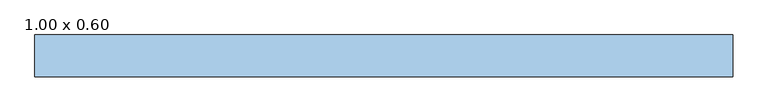
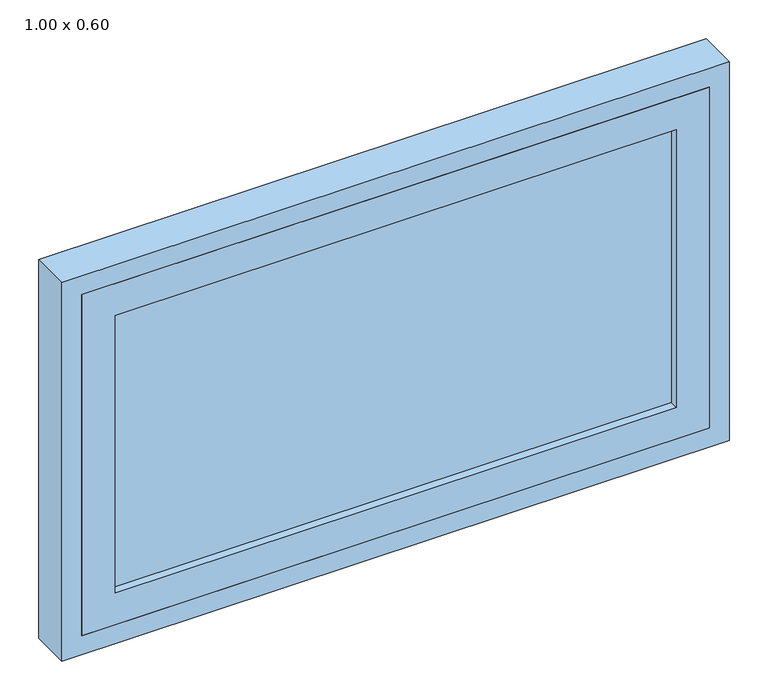
"""IFC4 building model written with IfcOpenShell, lengths in millimetres: window geometry, CC_JANELA MAXIM-AR_1 FOLHA VIDRO : 1.00 x 0.60."""

from ifc_helpers import new_model, si_unit, frame, origin, place, context, project, spatial, polyline, outline, extrude, source, transform, mapped, element, save


def window_1_00_x_0_60_42424789(model_context):
    return source(origin(), model_context, "Body", "SweptSolid", [
        extrude(outline(polyline([(-420.0, -87.5), (-420.0, -82.5), (420.0, -82.5), (420.0, -87.5), (-420.0, -87.5)])), frame((0.0, 0.0, 1780.0), z_axis=(0.0, 0.0, 1.0), x_axis=(1.0, 0.0, 0.0)), (0.0, 0.0, 1.0), 440.0),
        extrude(outline(polyline([(2270.0, -470.0), (1730.0, -470.0), (1730.0, 470.0), (2270.0, 470.0), (2270.0, -470.0)]), holes=[polyline([(2220.0, 420.0), (1780.0, 420.0), (1780.0, -420.0), (2220.0, -420.0), (2220.0, 420.0)])]), frame((0.0, -100.0, 0.0), z_axis=(0.0, 1.0, 0.0), x_axis=(0.0, 0.0, 1.0)), (0.0, 0.0, 1.0), 30.0),
        extrude(outline(polyline([(1700.0, 500.0), (2300.0, 500.0), (2300.0, -500.0), (1700.0, -500.0), (1700.0, 500.0)]), holes=[polyline([(1730.0, -470.0), (2270.0, -470.0), (2270.0, 470.0), (1730.0, 470.0), (1730.0, -470.0)])]), frame((0.0, -100.0, 0.0), z_axis=(0.0, 1.0, 0.0), x_axis=(0.0, 0.0, 1.0)), (0.0, 0.0, 1.0), 60.0),
    ])


if __name__ == "__main__":
    model = new_model("IFC4")
    model_context = context("Model", 3, world=origin())
    ifc_project = project(units=[si_unit("LENGTHUNIT", "METRE", prefix="MILLI")], contexts=[model_context])
    site = spatial("IfcSite", under=ifc_project)
    building = spatial("IfcBuilding", under=site)
    placement = place(None, origin())
    window_1_00_x_0_60_shape = window_1_00_x_0_60_42424789(model_context)
    element("IfcWindow", 1, ObjectType="CC_JANELA MAXIM-AR_1 FOLHA VIDRO : 1.00 x 0.60", at=placement, inside=building, context=model_context, shape_type="MappedRepresentation", body=[
        mapped(window_1_00_x_0_60_shape, transform((0.0, 0.0, 0.0), x_axis=(1.0, 0.0, 0.0), y_axis=(0.0, 1.0, 0.0), z_axis=(0.0, 0.0, 1.0))),
    ])
    save(model, "model.ifc")

# Revit data of these elements
# Type "CC_JANELA MAXIM-AR_1 FOLHA VIDRO : 1.00 x 0.60"
#   Type Mark = "J6"
#   Site = "www.construir.arq.br"
#   Empresa = "Cursos Construir"
#   Description = "JANELA MAXIM-AR 1 FOLHA VIDRO"
#   Criado Por = "Roberto Netto"
#   Analytic Construction = "<Nenhum>"
#   Atualizado por = "Rudemberg Eloi"
#   Rough Width = 1.00 m
#   Largura Moldura Folha [instance default] = 0.05 m
#   Largura Moldura Externa [instance default] = 0.10 m
#   Largura Guarnição Interna [instance default] = 0.05 m
#   Largura Folha [instance default] = 0.94 m
#   Interna [instance default] = 0.00 m
#   Externa [instance default] = 0.00 m
#   Extensão Frontal Peitoril/Pngadeira [instance default] = 0.03 m
#   Extensão Exterior Direita Peitoril/Pingadeira [instance default] = 0.025 m
#   Extensão Caixilho [instance default] = 0.03 m
#   Extensâo Exterior Esquerda Peitoril/Pingadeira [instance default] = 0.025 m
#   Espessura Peitoril/Pingadeira [instance default] = 0.02 m
#   Espessura Moldura Externa [instance default] = 0.01 m
#   Espessura Guarnição Interna [instance default] = 0.005 m
#   Espessura Folha [instance default] = 0.03 m
#   Espessura Caixilho [instance default] = 0.03 m
#   Cálculo Abertura Linear [instance default] = 0.00 m
#   Rough Height = 0.60 m
#   Altura Folha [instance default] = 0.54 m
#   Altura Corte [instance default] = 0.02 m
#   Height = 0.60 m
#   Width = 1.00 m
#   ----PEITORIL/PINGADEIRA---- [instance default] = 0.00 m
#   ----MOLDURA---- [instance default] = 0.00 m
#   ----GUARNIÇÃO---- [instance default] = 0.00 m
#   ----FOLHA---- [instance default] = 0.00 m
#   ----EXTENSÃO---- [instance default] = 0.00 m
#   ----CAIXILHO---- [instance default] = 0.00 m
#   Peitoril/Pingadeira Vazio [instance default] = no
#   Peitoril/Pingadeira Família [instance default] = yes
#   Moldura Externa [instance default] = no
#   Guarnição Interna [instance default] = yes
#   Material Vidro Folha = .VIDRO
#   Material Peitoril/Pingadeira = .GRANITO BRANCO ITAÚNAS
#   Material Moldura Folha = .ALUMÍNIO COM PINTURA ELETROSTÁTICA BRANCA
#   Material Moldura Externa = .PINTURA ACRÍLICA BRANCA
#   Material Guarnição = .ALUMÍNIO COM PINTURA ELETROSTÁTICA BRANCA
#   Material Caixilho = .ALUMÍNIO COM PINTURA ELETROSTÁTICA BRANCA
#   Wall Closure = (empty or 0)
# Element 1 (IfcWindow, "CC_JANELA MAXIM-AR_1 FOLHA VIDRO : 1.00 x 0.60")
#   Guarnição Interna = no
#   Materials on its faces: ".ALUMÍNIO COM PINTURA ELETROSTÁTICA BRANCA", ".VIDRO"
# Materials
#   ".VIDRO": class "Genérico", colour RGB 198 236 255, transparency 0.95, Cost = 0
#   ".GRANITO BRANCO ITAÚNAS": class ".CC_PEDRA REVEST.", colour RGB 202 195 174, transparency 0, Description = "Granito branco Itaúnas", Uso = "Pedra", Cost = 0
#   ".ALUMÍNIO COM PINTURA ELETROSTÁTICA BRANCA": class "CC_METAIS", colour RGB 241 241 241, transparency 0, Cost = 0
#   ".PINTURA ACRÍLICA BRANCA": class ".CC_PINTURA", colour RGB 250 250 250, transparency 0, Keynote = "09910.A1", Description = "Tinta acrílica na cor branca", Cost = 0
